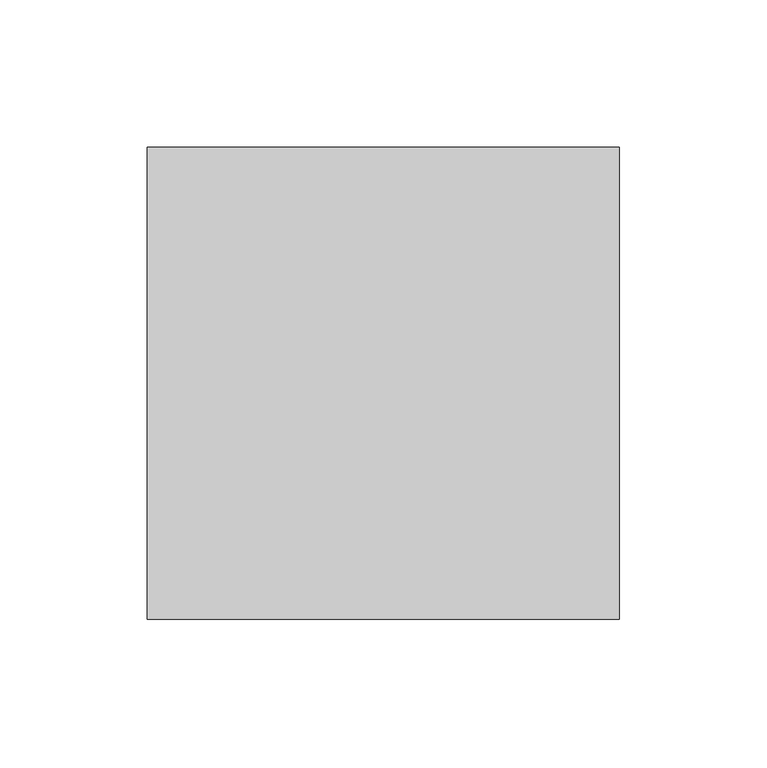
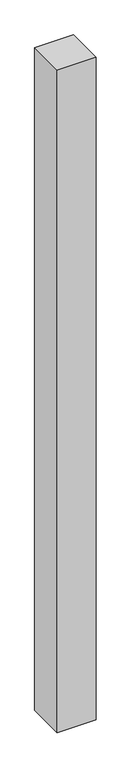
"""IFC4 building model written with IfcOpenShell, lengths in millimetres: proxy geometry, tjuk."""

from ifc_helpers import new_model, si_unit, origin, origin_with_axes, place, context, project, spatial, polyline, outline, extrude, source, transform, mapped, element, save


def generic_models_feebdf51(model_context):
    return source(origin(), model_context, "Body", "SweptSolid", [
        extrude(outline(polyline([(159076.7593015, 35937.2962965), (159076.7593015, 35777.2962965), (158916.7593015, 35777.2962965), (158916.7593015, 35937.2962965), (159076.7593015, 35937.2962965)])), origin_with_axes(), (0.0, 0.0, 1.0), 2880.0),
    ])


if __name__ == "__main__":
    model = new_model("IFC4")
    model_context = context("Model", 3, world=origin())
    ifc_project = project(units=[si_unit("LENGTHUNIT", "METRE", prefix="MILLI")], contexts=[model_context])
    site = spatial("IfcSite", under=ifc_project)
    building = spatial("IfcBuilding", under=site)
    placement = place(None, origin())
    generic_models_shape = generic_models_feebdf51(model_context)
    element("IfcBuildingElementProxy", 1, Name="tjuk", ObjectType="tjuk", at=placement, inside=building, context=model_context, shape_type="MappedRepresentation", body=[
        mapped(generic_models_shape, transform((0.0, 0.0, 0.0), x_axis=(1.0, 0.0, 0.0), y_axis=(0.0, 1.0, 0.0), z_axis=(0.0, 0.0, 1.0))),
    ])
    save(model, "model.ifc")

# Revit data of these elements
# Element 1 (IfcBuildingElementProxy, "tjuk")
#   Materials on its faces: "material wardrobe b 1"
# Materials
#   "material wardrobe b 1": class "Unassigned", colour RGB 128 128 128, transparency 0
